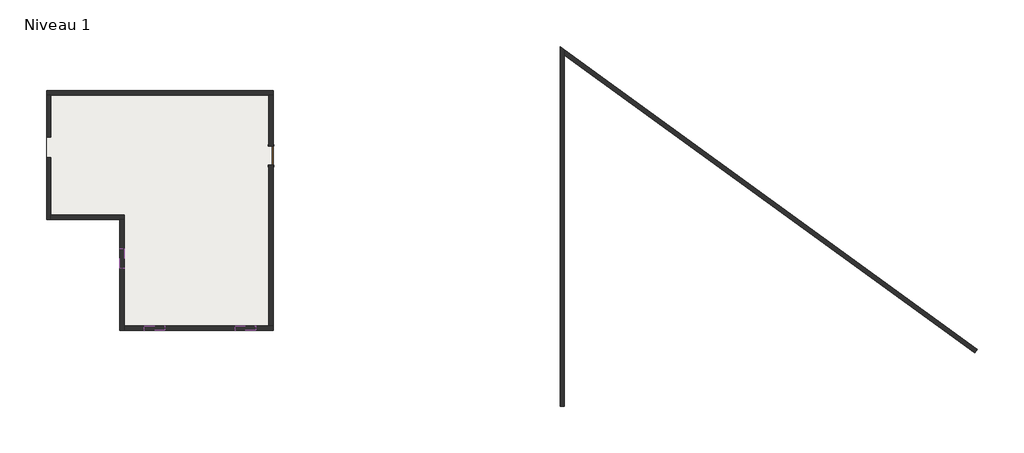
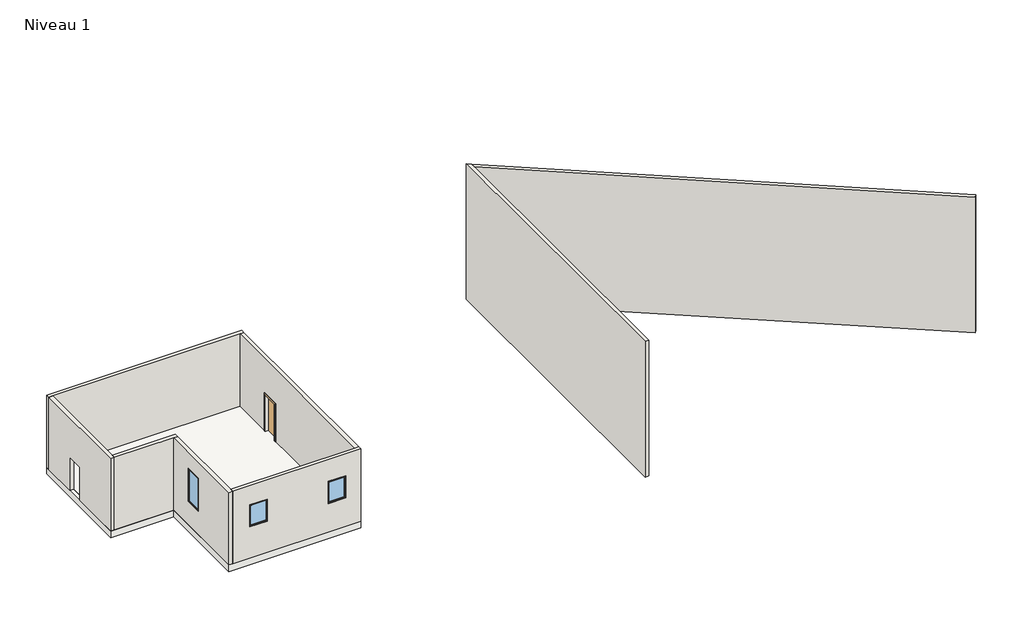
# One storey: 8 walls, 3 windows, 2 slabs, 1 door.
"""IFC4 building model written with IfcOpenShell, lengths in millimetres."""

import ifcopenshell
import ifcopenshell.guid

model = None  # the IFC model being written
_history = None  # IfcOwnerHistory: only IFC2X3 demands one
_inside = {}  # id of a spatial element -> (the spatial element, [elements in it])
_under = {}  # id of a project, library or spatial element -> (it, [spatial elements below it])
_declared = {}  # id of a project -> (the project, [libraries it declares])
_typed = {}  # id of a type object -> (the type object, [elements of that type])
_made_of = {}  # id of a material, layer set ... -> (it, [elements and type objects made of it])


def new_model(schema):
    """Start an empty IFC model of exactly this schema.

    Asked for "IFC4X3", IfcOpenShell would pick the latest addendum, in which some entities
    have other attributes; the version numbers below select the first issue.
    IFC2X3 requires an IfcOwnerHistory on every rooted entity: one is made here for all.
    """
    global model, _history
    if schema == "IFC4X3":
        model = ifcopenshell.file(schema_version=(4, 3, 0, 0))
    else:
        model = ifcopenshell.file(schema=schema)
    _inside.clear()
    _under.clear()
    _declared.clear()
    _typed.clear()
    _made_of.clear()
    _history = None
    if model.schema == "IFC2X3":
        org = make("IfcOrganization", Name="unknown")
        user = make(
            "IfcPersonAndOrganization",
            ThePerson=make("IfcPerson", FamilyName="unknown"),
            TheOrganization=org,
        )
        app = make(
            "IfcApplication",
            ApplicationDeveloper=org,
            Version="unknown",
            ApplicationFullName="unknown",
            ApplicationIdentifier="unknown",
        )
        _history = make(
            "IfcOwnerHistory",
            OwningUser=user,
            OwningApplication=app,
            ChangeAction="ADDED",
            CreationDate=0,
        )
    return model


def make(cls, **values):
    """One entity of the class cls with the attributes given. An attribute that is None is left unset."""
    return model.create_entity(
        cls, **{name: value for name, value in values.items() if value is not None}
    )


def rooted(cls, **values):
    """An entity with a GlobalId (a new one), such as an element, a storey or a relation."""
    return make(cls, GlobalId=ifcopenshell.guid.new(), OwnerHistory=_history, **values)


def si_unit(unit_type, name, prefix=None):
    """IfcSIUnit, for example si_unit("LENGTHUNIT", "METRE", prefix="MILLI")."""
    return make("IfcSIUnit", UnitType=unit_type, Prefix=prefix, Name=name)


def assignment(units):
    """IfcUnitAssignment: the units of a project."""
    return None if units is None else make("IfcUnitAssignment", Units=units)


def point(xyz):
    """IfcCartesianPoint."""
    return None if xyz is None else make("IfcCartesianPoint", Coordinates=xyz)


def direction(xyz):
    """IfcDirection."""
    return None if xyz is None else make("IfcDirection", DirectionRatios=xyz)


def frame(location, z_axis=None, x_axis=None):
    """IfcAxis2Placement3D, a coordinate frame: its origin and axes. An axis left out is left unset."""
    return make(
        "IfcAxis2Placement3D",
        Location=point(location),
        Axis=direction(z_axis),
        RefDirection=direction(x_axis),
    )


def origin():
    """The frame at (0, 0, 0) with its axes left unset."""
    return frame((0.0, 0.0, 0.0))


def origin_with_axes():
    """The frame at (0, 0, 0) with the z axis (0, 0, 1) and the x axis (1, 0, 0) written out."""
    return frame((0.0, 0.0, 0.0), z_axis=(0.0, 0.0, 1.0), x_axis=(1.0, 0.0, 0.0))


def place(relative_to, where):
    """IfcLocalPlacement: puts the frame where relative to a parent placement (None: the world)."""
    return make(
        "IfcLocalPlacement", PlacementRelTo=relative_to, RelativePlacement=where
    )


def context(
    kind, dimensions, precision=None, world=None, true_north=None, identifier=None
):
    """IfcGeometricRepresentationContext, for example the 3D "Model" context."""
    return make(
        "IfcGeometricRepresentationContext",
        ContextIdentifier=identifier,
        ContextType=kind,
        CoordinateSpaceDimension=dimensions,
        Precision=precision,
        WorldCoordinateSystem=world,
        TrueNorth=true_north,
    )


def project(units=None, contexts=None):
    """IfcProject with its units and contexts."""
    return rooted(
        "IfcProject",
        Name="project",
        RepresentationContexts=contexts,
        UnitsInContext=assignment(units),
    )


def spatial(cls, under=None, at=None, **own):
    """A site, building, storey or space (cls), placed at a placement, below another one or the project."""
    s = rooted(cls, ObjectPlacement=at, **own)
    if under is not None:
        _under.setdefault(under.id(), (under, []))[1].append(s)
    return s


def polyline(points):
    """IfcPolyline through the points."""
    return make("IfcPolyline", Points=[point(p) for p in points])


def outline(outer, holes=None, kind="AREA"):
    """IfcArbitraryClosedProfileDef: a profile drawn as a closed curve; with holes, ...WithVoids."""
    if holes is None:
        return make("IfcArbitraryClosedProfileDef", ProfileType=kind, OuterCurve=outer)
    return make(
        "IfcArbitraryProfileDefWithVoids",
        ProfileType=kind,
        OuterCurve=outer,
        InnerCurves=holes,
    )


def extrude(swept, where, along, depth):
    """IfcExtrudedAreaSolid: the profile swept, set in the frame where, extruded along a direction by depth."""
    return make(
        "IfcExtrudedAreaSolid",
        SweptArea=swept,
        Position=where,
        ExtrudedDirection=direction(along),
        Depth=depth,
    )


def faces_of(points, faces, orient=None, outer=None):
    """IfcFace entities. A face is a list of loops; a loop is a list of indices into points, from 0.

    orient and outer hold one flag for each loop. By default every Orientation is true, the
    first loop of a face is its IfcFaceOuterBound and the others are IfcFaceBound.
    """
    made = []
    for i, loops in enumerate(faces):
        bounds = []
        for j, loop in enumerate(loops):
            is_outer = j == 0 if outer is None else outer[i][j]
            bounds.append(
                make(
                    "IfcFaceOuterBound" if is_outer else "IfcFaceBound",
                    Bound=make("IfcPolyLoop", Polygon=[points[k] for k in loop]),
                    Orientation=True if orient is None else orient[i][j],
                )
            )
        made.append(make("IfcFace", Bounds=bounds))
    return made


def faceted_brep(points, faces, orient=None, outer=None, voids=None):
    """IfcFacetedBrep: a solid bounded by flat faces; with voids (closed shells), ...WithVoids."""
    shared = [point(p) for p in points]
    hull = make("IfcClosedShell", CfsFaces=faces_of(shared, faces, orient, outer))
    if voids is None:
        return make("IfcFacetedBrep", Outer=hull)
    return make(
        "IfcFacetedBrepWithVoids",
        Outer=hull,
        Voids=[
            make(cls, CfsFaces=faces_of(shared, fs, o, b)) for cls, fs, o, b in voids
        ],
    )


def shape(context_of_items, identifier, shape_type, items):
    """IfcShapeRepresentation: the items that make up one representation, for example the "Body"."""
    return make(
        "IfcShapeRepresentation",
        ContextOfItems=context_of_items,
        RepresentationIdentifier=identifier,
        RepresentationType=shape_type,
        Items=items,
    )


def source(mapping_origin, context_of_items, identifier, shape_type, items):
    """IfcRepresentationMap: a shape defined once, which mapped items show again and again."""
    return make(
        "IfcRepresentationMap",
        MappingOrigin=mapping_origin,
        MappedRepresentation=shape(context_of_items, identifier, shape_type, items),
    )


def transform(
    local_origin,
    x_axis=None,
    y_axis=None,
    z_axis=None,
    scale=None,
    scale2=None,
    scale3=None,
    uniform=True,
):
    """IfcCartesianTransformationOperator3D, or its non-uniform kind. x_axis, y_axis, z_axis: its Axis1, 2, 3."""
    if uniform:
        return make(
            "IfcCartesianTransformationOperator3D",
            Axis1=direction(x_axis),
            Axis2=direction(y_axis),
            LocalOrigin=point(local_origin),
            Scale=scale,
            Axis3=direction(z_axis),
        )
    return make(
        "IfcCartesianTransformationOperator3DnonUniform",
        Axis1=direction(x_axis),
        Axis2=direction(y_axis),
        LocalOrigin=point(local_origin),
        Scale=scale,
        Axis3=direction(z_axis),
        Scale2=scale2,
        Scale3=scale3,
    )


def mapped(mapping_source, mapping_target):
    """IfcMappedItem: shows the shape of a source again, moved by a transform."""
    return make(
        "IfcMappedItem", MappingSource=mapping_source, MappingTarget=mapping_target
    )


def made_of(thing, what):
    """Note that an element or type object is made of a material, layer set ...; save() writes the relation."""
    if what is not None:
        _made_of.setdefault(what.id(), (what, []))[1].append(thing)
    return thing


def element(
    cls,
    number,
    at=None,
    inside=None,
    cuts=None,
    type_object=None,
    material=None,
    context=None,
    identifier="Body",
    shape_type=None,
    held_by="IfcProductDefinitionShape",
    body=None,
    shapes=None,
    **own,
):
    """One element of the class cls, such as IfcWall. Its Tag is "e" and its number.

    at: its placement. inside: the storey or other place that contains it. cuts: it is an
    opening in that element (IfcRelVoidsElement). A single representation is given by context,
    identifier, shape_type and body (its items); several are given by shapes. held_by: the class
    of the entity that holds the representations. save() writes the other relations.
    """
    e = rooted(cls, Tag="e%d" % number, ObjectPlacement=at, **own)
    if body is not None:
        shapes = [shape(context, identifier, shape_type, body)]
    if shapes is not None:
        e.Representation = make(held_by, Representations=shapes)
    if inside is not None:
        _inside.setdefault(inside.id(), (inside, []))[1].append(e)
    if cuts is not None:
        rooted(
            "IfcRelVoidsElement", RelatingBuildingElement=cuts, RelatedOpeningElement=e
        )
    if type_object is not None:
        _typed.setdefault(type_object.id(), (type_object, []))[1].append(e)
    return made_of(e, material)


def aggregate(whole, parts):
    """IfcRelAggregates: a whole, such as a stair, and the parts it consists of."""
    return rooted("IfcRelAggregates", RelatingObject=whole, RelatedObjects=parts)


def save(model, path):
    """Write the relations noted so far, then the file.

    IfcRelAggregates (storeys below a building ...), IfcRelContainedInSpatialStructure (elements
    in a storey), IfcRelDefinesByType, IfcRelAssociatesMaterial and IfcRelDeclares: one each for
    every whole, place, type object, material and project.
    """
    for whole, parts in _under.values():
        aggregate(whole, parts)
    for where, things in _inside.values():
        rooted(
            "IfcRelContainedInSpatialStructure",
            RelatedElements=things,
            RelatingStructure=where,
        )
    for kind, things in _typed.values():
        rooted("IfcRelDefinesByType", RelatedObjects=things, RelatingType=kind)
    for what, things in _made_of.values():
        rooted("IfcRelAssociatesMaterial", RelatedObjects=things, RelatingMaterial=what)
    for by, libraries in _declared.values():
        rooted("IfcRelDeclares", RelatingContext=by, RelatedDefinitions=libraries)
    model.write(path)


def simple_avec_alignement_0864_x_2032mm_aeff3166(model_context):
    return source(origin(), model_context, "Body", "SweptSolid", [
        extrude(outline(polyline([(2108.0, -508.0), (0.0, -508.0), (0.0, -432.0), (2032.0, -432.0), (2032.0, 432.0), (0.0, 432.0), (0.0, 508.0), (2108.0, 508.0), (2108.0, -508.0)])), frame((0.0, 100.0, 0.0), z_axis=(0.0, 1.0, 0.0), x_axis=(0.0, 0.0, 1.0)), (0.0, 0.0, 1.0), 25.0),
        extrude(outline(polyline([(2108.0, 508.0), (2108.0, -508.0), (0.0, -508.0), (0.0, -432.0), (2032.0, -432.0), (2032.0, 432.0), (0.0, 432.0), (0.0, 508.0), (2108.0, 508.0)])), frame((0.0, -125.0, 0.0), z_axis=(0.0, 1.0, 0.0), x_axis=(0.0, 0.0, 1.0)), (0.0, 0.0, 1.0), 25.0),
        extrude(outline(polyline([(432.0, 49.0), (-432.0, 49.0), (-432.0, 100.0), (432.0, 100.0), (432.0, 49.0)])), origin_with_axes(), (0.0, 0.0, 1.0), 2032.0),
    ])


def fixe_0915_x_1220mm_488fb2fb(model_context):
    return source(origin(), model_context, "Body", "SweptSolid", [
        extrude(outline(polyline([(-394.5, 78.0), (394.5, 78.0), (394.5, 66.0), (-394.5, 66.0), (-394.5, 78.0)])), frame((0.0, 0.0, 978.0), z_axis=(0.0, 0.0, 1.0), x_axis=(1.0, 0.0, 0.0)), (0.0, 0.0, 1.0), 1094.0),
        extrude(outline(polyline([(2116.0, -438.5), (934.0, -438.5), (934.0, 438.5), (2116.0, 438.5), (2116.0, -438.5)]), holes=[polyline([(2072.0, -394.5), (2072.0, 394.5), (978.0, 394.5), (978.0, -394.5), (2072.0, -394.5)])]), frame((0.0, 50.0, 0.0), z_axis=(0.0, 1.0, 0.0), x_axis=(0.0, 0.0, 1.0)), (0.0, 0.0, 1.0), 44.0),
        extrude(outline(polyline([(2135.0, -457.5), (915.0, -457.5), (915.0, 457.5), (2135.0, 457.5), (2135.0, -457.5)]), holes=[polyline([(2116.0, -438.5), (2116.0, 438.5), (934.0, 438.5), (934.0, -438.5), (2116.0, -438.5)])]), frame((0.0, 50.0, 0.0), z_axis=(0.0, 1.0, 0.0), x_axis=(0.0, 0.0, 1.0)), (0.0, 0.0, 1.0), 63.0),
        extrude(outline(polyline([(2135.0, -457.5), (915.0, -457.5), (915.0, 457.5), (2135.0, 457.5), (2135.0, -457.5)]), holes=[polyline([(2103.0, -425.5), (2103.0, 425.5), (947.0, 425.5), (947.0, -425.5), (2103.0, -425.5)])]), frame((0.0, -87.0, 0.0), z_axis=(0.0, 1.0, 0.0), x_axis=(0.0, 0.0, 1.0)), (0.0, 0.0, 1.0), 137.0),
    ])


def fixe_0915_x_1830mm_5d6e8bc1(model_context):
    return source(origin(), model_context, "Body", "SweptSolid", [
        extrude(outline(polyline([(-394.5, 78.0), (394.5, 78.0), (394.5, 66.0), (-394.5, 66.0), (-394.5, 78.0)])), frame((0.0, 0.0, 368.0), z_axis=(0.0, 0.0, 1.0), x_axis=(1.0, 0.0, 0.0)), (0.0, 0.0, 1.0), 1704.0),
        extrude(outline(polyline([(2116.0, -438.5), (324.0, -438.5), (324.0, 438.5), (2116.0, 438.5), (2116.0, -438.5)]), holes=[polyline([(2072.0, -394.5), (2072.0, 394.5), (368.0, 394.5), (368.0, -394.5), (2072.0, -394.5)])]), frame((0.0, 50.0, 0.0), z_axis=(0.0, 1.0, 0.0), x_axis=(0.0, 0.0, 1.0)), (0.0, 0.0, 1.0), 44.0),
        extrude(outline(polyline([(2135.0, -457.5), (305.0, -457.5), (305.0, 457.5), (2135.0, 457.5), (2135.0, -457.5)]), holes=[polyline([(2116.0, -438.5), (2116.0, 438.5), (324.0, 438.5), (324.0, -438.5), (2116.0, -438.5)])]), frame((0.0, 50.0, 0.0), z_axis=(0.0, 1.0, 0.0), x_axis=(0.0, 0.0, 1.0)), (0.0, 0.0, 1.0), 63.0),
        extrude(outline(polyline([(2135.0, -457.5), (305.0, -457.5), (305.0, 457.5), (2135.0, 457.5), (2135.0, -457.5)]), holes=[polyline([(2103.0, -425.5), (2103.0, 425.5), (337.0, 425.5), (337.0, -425.5), (2103.0, -425.5)])]), frame((0.0, -87.0, 0.0), z_axis=(0.0, 1.0, 0.0), x_axis=(0.0, 0.0, 1.0)), (0.0, 0.0, 1.0), 137.0),
    ])


model = new_model("IFC4")

# Units and contexts
model_context = context("Model", 3, world=origin())
ifc_project = project(units=[si_unit("LENGTHUNIT", "METRE", prefix="MILLI")], contexts=[model_context])

# Site, building, storey
site = spatial("IfcSite", under=ifc_project)
building = spatial("IfcBuilding", under=site)
storey = spatial("IfcBuildingStorey", under=building, Name="Niveau 1", Elevation=0.0)

# Door
placement = place(None, origin())
simple_avec_alignement_0864_x_2032mm_shape = simple_avec_alignement_0864_x_2032mm_aeff3166(model_context)
element("IfcDoor", 1, ObjectType="Simple avec alignement : 0864 x 2032mm", at=placement, inside=storey, context=model_context, shape_type="MappedRepresentation", body=[
    mapped(simple_avec_alignement_0864_x_2032mm_shape, transform((4978.3276717, 1507.3554467, 0.0), x_axis=(0.0, -1.0, 0.0), y_axis=(1.0, 0.0, 0.0), z_axis=(0.0, 0.0, 1.0))),
])

# Slabs
element("IfcSlab", 2, ObjectType="Béton - Commercial 362 mm", at=placement, inside=storey, context=model_context, shape_type="SweptSolid", body=[
    extrude(outline(polyline([(5078.3276717, 4439.3554467), (5078.3276717, -6360.6445533), (-1821.6723283, -6360.6445533), (-1821.6723283, -1360.6445533), (-5121.6723283, -1360.6445533), (-5121.6723283, 4439.3554467), (5078.3276717, 4439.3554467)])), frame((0.0, 0.0, -362.0), z_axis=(0.0, 0.0, 1.0), x_axis=(1.0, 0.0, 0.0)), (0.0, 0.0, 1.0), 362.0),
])
element("IfcSlab", 3, ObjectType="Béton - Commercial 362 mm", at=placement, inside=storey, context=model_context, shape_type="SweptSolid", body=[
    extrude(outline(polyline([(4878.3276717, 4239.3554467), (4878.3276717, -6160.6445533), (-1621.6723283, -6160.6445533), (-1621.6723283, -1160.6445533), (-4921.6723283, -1160.6445533), (-4921.6723283, 4239.3554467), (4878.3276717, 4239.3554467)])), frame((0.0, 0.0, -362.0), z_axis=(0.0, 0.0, 1.0), x_axis=(1.0, 0.0, 0.0)), (0.0, 0.0, 1.0), 362.0),
])

# Walls
element("IfcWall", 4, ObjectType="Générique - 200 mm", at=placement, inside=storey, context=model_context, shape_type="Brep", body=[
    faceted_brep([(-5121.6723283, 4239.3554467, 0.0), (-4921.6723283, 4239.3554467, 0.0), (4878.3276717, 4239.3554467, 0.0), (5078.3276717, 4239.3554467, 0.0), (5078.3276717, 4239.3554467, 4000.0), (4878.3276717, 4239.3554467, 4000.0), (-4921.6723283, 4239.3554467, 4000.0), (-5121.6723283, 4239.3554467, 4000.0), (-5121.6723283, 4439.3554467, 0.0), (-5121.6723283, 4439.3554467, 4000.0), (5078.3276717, 4439.3554467, 4000.0), (5078.3276717, 4439.3554467, 0.0)], [[[0, 1, 2, 3, 4, 5, 6, 7]], [[8, 9, 10, 11]], [[3, 2, 1, 0, 8, 11]], [[7, 6, 5, 4, 10, 9]], [[0, 7, 9, 8]], [[4, 3, 11, 10]]]),
])
element("IfcWall", 5, ObjectType="Générique - 200 mm", at=placement, inside=storey, context=model_context, shape_type="Brep", body=[
    faceted_brep([(-5121.6723283, -1360.6445533, 4000.0), (-5121.6723283, 4239.3554467, 4000.0), (-5121.6723283, 4239.3554467, 0.0), (-5121.6723283, 2339.3554467, 0.0), (-5121.6723283, 2339.3554467, 1834.0), (-5121.6723283, 1424.3554467, 1834.0), (-5121.6723283, 1424.3554467, 0.0), (-5121.6723283, -1360.6445533, 0.0), (-4921.6723283, 4239.3554467, 4000.0), (-4921.6723283, -1160.6445533, 4000.0), (-4921.6723283, -1360.6445533, 4000.0), (-4921.6723283, -1360.6445533, 0.0), (-4921.6723283, -1160.6445533, 0.0), (-4921.6723283, 1424.3554467, 0.0), (-4921.6723283, 1424.3554467, 1834.0), (-4921.6723283, 2339.3554467, 1834.0), (-4921.6723283, 2339.3554467, 0.0), (-4921.6723283, 4239.3554467, 0.0)], [[[0, 1, 2, 3, 4, 5, 6, 7]], [[8, 9, 10, 11, 12, 13, 14, 15, 16, 17]], [[2, 17, 16, 3]], [[11, 7, 6, 13, 12]], [[1, 0, 10, 9, 8]], [[2, 1, 8, 17]], [[0, 7, 11, 10]], [[15, 4, 3, 16]], [[4, 15, 14, 5]], [[5, 14, 13, 6]]]),
])
element("IfcWall", 6, ObjectType="Générique - 200 mm", at=placement, inside=storey, context=model_context, shape_type="Brep", body=[
    faceted_brep([(-4921.6723283, -1360.6445533, 0.0), (-1821.6723283, -1360.6445533, 0.0), (-1621.6723283, -1360.6445533, 0.0), (-1621.6723283, -1360.6445533, 4000.0), (-1821.6723283, -1360.6445533, 4000.0), (-4921.6723283, -1360.6445533, 4000.0), (-4921.6723283, -1160.6445533, 0.0), (-4921.6723283, -1160.6445533, 4000.0), (-1621.6723283, -1160.6445533, 4000.0), (-1621.6723283, -1160.6445533, 0.0)], [[[0, 1, 2, 3, 4, 5]], [[6, 7, 8, 9]], [[2, 1, 0, 6, 9]], [[5, 4, 3, 8, 7]], [[0, 5, 7, 6]], [[3, 2, 9, 8]]]),
])
element("IfcWall", 7, ObjectType="Générique - 200 mm", at=placement, inside=storey, context=model_context, shape_type="Brep", body=[
    faceted_brep([(-1821.6723283, -1360.6445533, 0.0), (-1821.6723283, -6360.6445533, 0.0), (-1821.6723283, -6360.6445533, 4000.0), (-1821.6723283, -1360.6445533, 4000.0), (-1821.6723283, -3575.6445533, 1279.9492891), (-1821.6723283, -2660.6445533, 1279.9492891), (-1821.6723283, -2660.6445533, 3109.9492891), (-1821.6723283, -3575.6445533, 3109.9492891), (-1621.6723283, -1360.6445533, 0.0), (-1621.6723283, -1360.6445533, 4000.0), (-1621.6723283, -6160.6445533, 4000.0), (-1621.6723283, -6360.6445533, 4000.0), (-1621.6723283, -6360.6445533, 0.0), (-1621.6723283, -6160.6445533, 0.0), (-1621.6723283, -3575.6445533, 1279.9492891), (-1621.6723283, -3575.6445533, 3109.9492891), (-1621.6723283, -2660.6445533, 3109.9492891), (-1621.6723283, -2660.6445533, 1279.9492891)], [[[0, 1, 2, 3], [4, 5, 6, 7]], [[8, 9, 10, 11, 12, 13], [14, 15, 16, 17]], [[1, 0, 8, 13, 12]], [[3, 2, 11, 10, 9]], [[0, 3, 9, 8]], [[2, 1, 12, 11]], [[15, 14, 4, 7]], [[16, 15, 7, 6]], [[17, 16, 6, 5]], [[14, 17, 5, 4]]]),
])
element("IfcWall", 8, ObjectType="Générique - 200 mm", at=placement, inside=storey, context=model_context, shape_type="Brep", body=[
    faceted_brep([(-1621.6723283, -6360.6445533, 0.0), (5078.3276717, -6360.6445533, 0.0), (5078.3276717, -6360.6445533, 4000.0), (-1621.6723283, -6360.6445533, 4000.0), (4278.3276717, -6360.6445533, 1581.4154575), (3363.3276717, -6360.6445533, 1581.4154575), (3363.3276717, -6360.6445533, 2801.4154575), (4278.3276717, -6360.6445533, 2801.4154575), (193.3276717, -6360.6445533, 1720.4721695), (-721.6723283, -6360.6445533, 1720.4721695), (-721.6723283, -6360.6445533, 2940.4721695), (193.3276717, -6360.6445533, 2940.4721695), (-1621.6723283, -6160.6445533, 0.0), (-1621.6723283, -6160.6445533, 4000.0), (4878.3276717, -6160.6445533, 4000.0), (5078.3276717, -6160.6445533, 4000.0), (5078.3276717, -6160.6445533, 0.0), (4878.3276717, -6160.6445533, 0.0), (4278.3276717, -6160.6445533, 1581.4154575), (4278.3276717, -6160.6445533, 2801.4154575), (3363.3276717, -6160.6445533, 2801.4154575), (3363.3276717, -6160.6445533, 1581.4154575), (193.3276717, -6160.6445533, 1720.4721695), (193.3276717, -6160.6445533, 2940.4721695), (-721.6723283, -6160.6445533, 2940.4721695), (-721.6723283, -6160.6445533, 1720.4721695)], [[[0, 1, 2, 3], [4, 5, 6, 7], [8, 9, 10, 11]], [[12, 13, 14, 15, 16, 17], [18, 19, 20, 21], [22, 23, 24, 25]], [[1, 0, 12, 17, 16]], [[3, 2, 15, 14, 13]], [[0, 3, 13, 12]], [[2, 1, 16, 15]], [[19, 18, 4, 7]], [[20, 19, 7, 6]], [[21, 20, 6, 5]], [[18, 21, 5, 4]], [[23, 22, 8, 11]], [[24, 23, 11, 10]], [[25, 24, 10, 9]], [[22, 25, 9, 8]]]),
])
element("IfcWall", 9, ObjectType="Générique - 200 mm", at=placement, inside=storey, context=model_context, shape_type="SweptSolid", body=[
    extrude(outline(polyline([(1075.3554467, 2032.0), (1075.3554467, 0.0), (-6160.6445533, 0.0), (-6160.6445533, 4000.0), (4239.3554467, 4000.0), (4239.3554467, 0.0), (1939.3554467, 0.0), (1939.3554467, 2032.0), (1075.3554467, 2032.0)])), frame((4878.3276717, 0.0, 0.0), z_axis=(1.0, 0.0, 0.0), x_axis=(0.0, 1.0, 0.0)), (0.0, 0.0, 1.0), 200.0),
])
element("IfcWall", 10, ObjectType="Générique - 200 mm", at=placement, inside=storey, context=model_context, shape_type="Brep", body=[
    faceted_brep([(18162.9994118, -9776.735206, 0.0), (18162.9994118, 6027.0037435, 0.0), (18162.9994118, 6274.217339, 0.0), (18162.9994118, 6274.217339, 7500.0), (18162.9994118, 6027.0037435, 7500.0), (18162.9994118, -9776.735206, 7500.0), (17962.9994118, -9776.735206, 0.0), (17962.9994118, -9776.735206, 7500.0), (17962.9994118, 6419.5258446, 7500.0), (17962.9994118, 6419.5258446, 0.0)], [[[0, 1, 2, 3, 4, 5]], [[6, 7, 8, 9]], [[2, 1, 0, 6, 9]], [[5, 4, 3, 8, 7]], [[0, 5, 7, 6]], [[3, 2, 9, 8]]]),
])
element("IfcWall", 11, ObjectType="Générique - 200 mm", at=placement, inside=storey, context=model_context, shape_type="SweptSolid", body=[
    extrude(outline(polyline([(36611.6117571, -7376.6977082), (18162.9994118, 6027.0037435), (18162.9994118, 6274.217339), (36729.1688076, -7214.8943093), (36611.6117571, -7376.6977082)])), origin_with_axes(), (0.0, 0.0, 1.0), 7500.0),
])

# Windows
fixe_0915_x_1220mm_shape = fixe_0915_x_1220mm_488fb2fb(model_context)
element("IfcWindow", 12, ObjectType="Fixe : 0915 x 1220mm", at=placement, inside=storey, context=model_context, shape_type="MappedRepresentation", body=[
    mapped(fixe_0915_x_1220mm_shape, transform((3820.8276717, -6247.6445533, 666.4154575), x_axis=(-1.0, 0.0, 0.0), y_axis=(0.0, -1.0, 0.0), z_axis=(0.0, 0.0, 1.0))),
])
element("IfcWindow", 13, ObjectType="Fixe : 0915 x 1220mm", at=placement, inside=storey, context=model_context, shape_type="MappedRepresentation", body=[
    mapped(fixe_0915_x_1220mm_shape, transform((-264.1723283, -6247.6445533, 805.4721695), x_axis=(-1.0, 0.0, 0.0), y_axis=(0.0, -1.0, 0.0), z_axis=(0.0, 0.0, 1.0))),
])
fixe_0915_x_1830mm_shape = fixe_0915_x_1830mm_5d6e8bc1(model_context)
element("IfcWindow", 14, ObjectType="Fixe : 0915 x 1830mm", at=placement, inside=storey, context=model_context, shape_type="MappedRepresentation", body=[
    mapped(fixe_0915_x_1830mm_shape, transform((-1708.6723283, -3118.1445533, 974.9492891), x_axis=(0.0, 1.0, 0.0), y_axis=(-1.0, 0.0, 0.0), z_axis=(0.0, 0.0, 1.0))),
])

save(model, "model.ifc")

# Revit data of these elements
# Project information
#   Date de fin du projet = "Date de fin"
#   Etat du projet = "Etat du projet"
#   Nom du client = "Propriétaire"
#   Adresse du projet = "Entrer l'adresse ici"
#   Nom du projet = "Nom du projet"
#   Numéro de projet = "0001"
# Type "Simple avec alignement : 0864 x 2032mm"
#   Type Mark = "22"
#   Construction Type Id = "MDOOR"
#   Analytic Construction = "Métal"
#   Thickness = 0.051 m
#   Heat Transfer Coefficient (U) = 3.7021 W/(m²·K)
#   Height = 2.032 m
#   Ajuster la projection Ext = 0.025 m
#   Ajuster la projection Int = 0.025 m
#   Ajuster la largeur = 0.076 m
#   Width = 0.864 m
#   Function = 0
#   Define Thermal Properties by = 1
#   Matériau de porte = Porte - Panneau
#   Matériau des huisseries = Porte - Cadre
#   Visual Light Transmittance = 0
#   Solar Heat Gain Coefficient = 0
#   Function = (empty or 0)
#   Wall Closure = (empty or 0)
# Type "Béton - Commercial 362 mm"
#   Function = 0
#   Layers, outside or top first: 0.20 m "Béton, coulé sur place" (function 1); 0.00 m "Isolant imperméable" (function 100); 0.012 m "Sable" (function 0); 0.15 m "Site - Agrégats" (function 0)
# Type "Générique - 200 mm"
#   Layers, outside or top first: 0.20 m no material (function 1)
# Type "Fixe : 0915 x 1220mm"
#   Type Mark = "15"
#   Construction Type Id = "GSP4R"
#   Analytic Construction = "Simple vitrage Pilkington 1/8 po."
#   Visual Light Transmittance = 0.9
#   Solar Heat Gain Coefficient = 0.78
#   Heat Transfer Coefficient (U) = 3.6886 W/(m²·K)
#   Height = 1.22 m
#   Hauteur de l'appui par défaut = 0.915 m
#   Width = 0.915 m
#   Encastrement de fenêtre = 0.019 m
#   Define Thermal Properties by = 1
#   Matériau de cadre extérieur = Châssis
#   Matériau du cadre intérieur = Châssis
#   Matériau du panneau de verre = Verre
#   Châssis = Châssis
#   Wall Closure = (empty or 0)
# Type "Fixe : 0915 x 1830mm"
#   Type Mark = "18"
#   Construction Type Id = "GSP4R"
#   Analytic Construction = "Simple vitrage Pilkington 1/8 po."
#   Visual Light Transmittance = 0.9
#   Solar Heat Gain Coefficient = 0.78
#   Heat Transfer Coefficient (U) = 3.6886 W/(m²·K)
#   Height = 1.83 m
#   Hauteur de l'appui par défaut = 0.305 m
#   Width = 0.915 m
#   Encastrement de fenêtre = 0.019 m
#   Define Thermal Properties by = 1
#   Matériau de cadre extérieur = Châssis
#   Matériau du cadre intérieur = Châssis
#   Matériau du panneau de verre = Verre
#   Châssis = Châssis
#   Wall Closure = (empty or 0)
# Element 1 (IfcDoor, "Simple avec alignement : 0864 x 2032mm")
#   Phase Created = Phase 1
#   Materials on its faces: "Porte - Cadre", "Porte - Panneau"
# Element 2 (IfcSlab, "Béton - Commercial 362 mm")
#   Height Offset From Level = 0.00 m
#   built-in parameter 1001954 = 1
#   Phase Created = Phase 1
#   Materials on its faces: "Site - Agrégats", "Béton, coulé sur place"
# Element 3 (IfcSlab, "Béton - Commercial 362 mm")
#   Height Offset From Level = 0.00 m
#   Phase Created = Phase 1
#   Materials on its faces: "Site - Agrégats", "Béton, coulé sur place"
# Elements 4, 5, 6, 7, 9 (IfcWall, "Générique - 200 mm")
#   Top Offset = 0.00 m
#   Base Offset = 0.00 m
#   wall height = 4.00 m
#   Phase Created = Phase 1
#   Base Constraint = Niveau 1
#   Top Constraint = Niveau 2
#   Materials on its faces: "Mur par défaut"
# Element 8 (IfcWall, "Générique - 200 mm")
#   Top Offset = 0.00 m
#   Base Offset = 0.00 m
#   wall height = 4.00 m
#   Cout total = 688888
#   Cout unitaire = 30
#   Phase Created = Phase 1
#   Base Constraint = Niveau 1
#   Top Constraint = Niveau 2
#   Materials on its faces: "Mur par défaut"
# Elements 10, 11 (IfcWall, "Générique - 200 mm")
#   Top Offset = 0.00 m
#   Base Offset = 0.00 m
#   wall height = 7.50 m
#   Phase Created = Phase 1
#   Base Constraint = Niveau 1
#   Top Constraint = Niveau 3
#   Materials on its faces: "Mur par défaut"
# Element 12 (IfcWindow, "Fixe : 0915 x 1220mm")
#   Mark = "2"
#   Phase Created = Phase 1
#   Materials on its faces: "Châssis", "Verre"
# Element 13 (IfcWindow, "Fixe : 0915 x 1220mm")
#   Mark = "3"
#   Phase Created = Phase 1
#   Materials on its faces: "Châssis", "Verre"
# Element 14 (IfcWindow, "Fixe : 0915 x 1830mm")
#   Mark = "1"
#   Phase Created = Phase 1
#   Materials on its faces: "Châssis", "Verre"
# Materials
#   "Porte - Panneau": class "Bois", colour RGB 210 159 95, transparency 0, Cost = 0
#   "Porte - Cadre": class "Peinture", colour RGB 118 70 51, transparency 0, Cost = 0
#   "Béton, coulé sur place": class "Béton", colour RGB 192 192 192, transparency 0, Description = "Matériau physique", Cost = 0
#   "Isolant imperméable": class "Générique", colour RGB 127 127 127, transparency 0, Description = "Isolant imperméable", Cost = 0
#   "Sable": class "Générique", colour RGB 191 183 178, transparency 0, Description = "Sable", Cost = 0
#   "Site - Agrégats": class "Divers", colour RGB 165 42 42, transparency 0, Cost = 0
#   "Châssis": class "Bois", colour RGB 224 178 126, transparency 0, Cost = 0
#   "Verre": class "Verre", colour RGB 0 128 192, transparency 0.9, Description = "Verre sodocalcique", Cost = 0
#   "Mur par défaut": class "Divers", colour RGB 128 128 128, transparency 0, Cost = 0
